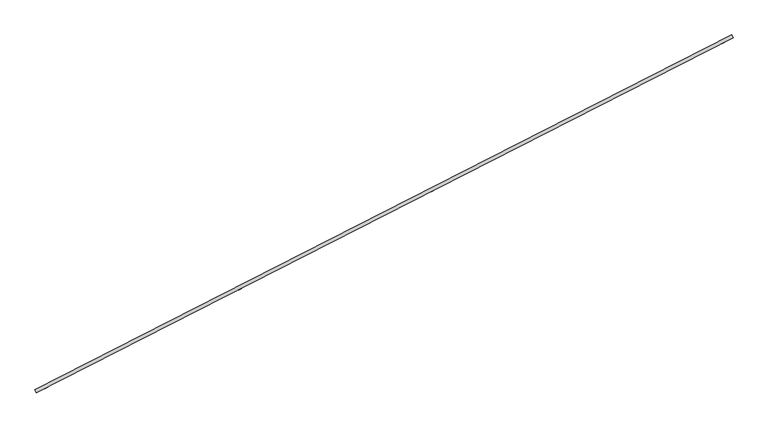
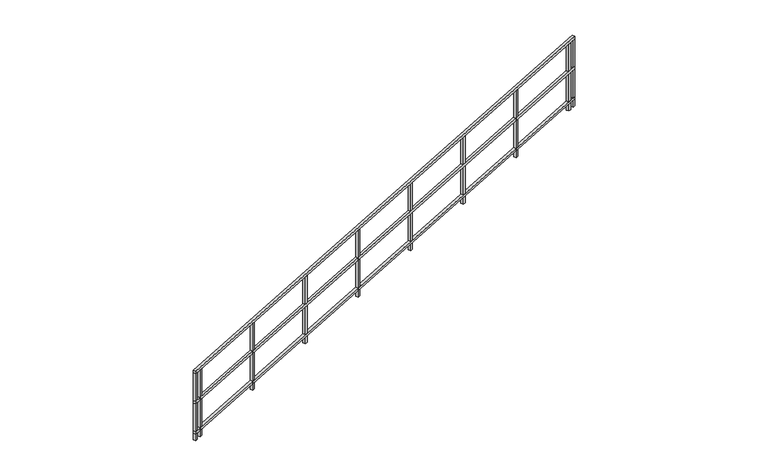
"""IFC4 building model written with IfcOpenShell, lengths in millimetres: railing geometry."""

from ifc_helpers import new_model, si_unit, frame, origin, place, context, project, spatial, polyline, outline, extrude, source, transform, mapped, element, save


def railing_8f82b1fa(model_context):
    return source(origin(), model_context, "Body", "SweptSolid", [
        extrude(outline(polyline([(54203.6748483, 45637.5924682), (54220.9718863, 45603.6451197), (46399.2676625, 41618.2877592), (46381.9706245, 41652.2351078), (54203.6748483, 45637.5924682)])), frame((0.0, 0.0, 266339.5064882), z_axis=(0.0, 0.0, 1.0), x_axis=(1.0, 0.0, 0.0)), (0.0, 0.0, 1.0), 38.1),
        extrude(outline(polyline([(54203.6748483, 45637.5924682), (54220.9718863, 45603.6451197), (46399.2676625, 41618.2877592), (46381.9706245, 41652.2351078), (54203.6748483, 45637.5924682)])), frame((0.0, 0.0, 265875.9564882), z_axis=(0.0, 0.0, 1.0), x_axis=(1.0, 0.0, 0.0)), (0.0, 0.0, 1.0), 38.1),
        extrude(outline(polyline([(54203.6748483, 45637.5924682), (54220.9718863, 45603.6451197), (46399.2676625, 41618.2877592), (46381.9706245, 41652.2351078), (54203.6748483, 45637.5924682)])), frame((0.0, 0.0, 265412.4064882), z_axis=(0.0, 0.0, 1.0), x_axis=(1.0, 0.0, 0.0)), (0.0, 0.0, 1.0), 38.1),
        extrude(outline(polyline([(46524.9904087, 41682.346698), (46491.0430601, 41665.0496599), (46473.7460221, 41698.9970085), (46507.6933706, 41716.2940465), (46524.9904087, 41682.346698)])), frame((0.0, 0.0, 265310.8064882), z_axis=(0.0, 0.0, 1.0), x_axis=(1.0, 0.0, 0.0)), (0.0, 0.0, 1.0), 1028.7),
        extrude(outline(polyline([(47611.305563, 42235.8519153), (47577.3582144, 42218.5548772), (47560.0611764, 42252.5022258), (47594.0085249, 42269.7992638), (47611.305563, 42235.8519153)])), frame((0.0, 0.0, 265310.8064882), z_axis=(0.0, 0.0, 1.0), x_axis=(1.0, 0.0, 0.0)), (0.0, 0.0, 1.0), 1028.7),
        extrude(outline(polyline([(48697.6207173, 42789.3571325), (48663.6733687, 42772.0600945), (48646.3763307, 42806.0074431), (48680.3236792, 42823.3044811), (48697.6207173, 42789.3571325)])), frame((0.0, 0.0, 265310.8064882), z_axis=(0.0, 0.0, 1.0), x_axis=(1.0, 0.0, 0.0)), (0.0, 0.0, 1.0), 1028.7),
        extrude(outline(polyline([(49783.9358716, 43342.8623498), (49749.988523, 43325.5653118), (49732.6914849, 43359.5126604), (49766.6388335, 43376.8096984), (49783.9358716, 43342.8623498)])), frame((0.0, 0.0, 265310.8064882), z_axis=(0.0, 0.0, 1.0), x_axis=(1.0, 0.0, 0.0)), (0.0, 0.0, 1.0), 1028.7),
        extrude(outline(polyline([(50870.2510258, 43896.3675671), (50836.3036773, 43879.0705291), (50819.0066392, 43913.0178776), (50852.9539878, 43930.3149157), (50870.2510258, 43896.3675671)])), frame((0.0, 0.0, 265310.8064882), z_axis=(0.0, 0.0, 1.0), x_axis=(1.0, 0.0, 0.0)), (0.0, 0.0, 1.0), 1028.7),
        extrude(outline(polyline([(51956.5661801, 44449.8727844), (51922.6188316, 44432.5757463), (51905.3217935, 44466.5230949), (51939.2691421, 44483.820133), (51956.5661801, 44449.8727844)])), frame((0.0, 0.0, 265310.8064882), z_axis=(0.0, 0.0, 1.0), x_axis=(1.0, 0.0, 0.0)), (0.0, 0.0, 1.0), 1028.7),
        extrude(outline(polyline([(53042.8813344, 45003.3780017), (53008.9339859, 44986.0809636), (52991.6369478, 45020.0283122), (53025.5842964, 45037.3253502), (53042.8813344, 45003.3780017)])), frame((0.0, 0.0, 265310.8064882), z_axis=(0.0, 0.0, 1.0), x_axis=(1.0, 0.0, 0.0)), (0.0, 0.0, 1.0), 1028.7),
        extrude(outline(polyline([(54129.1964887, 45556.883219), (54095.2491401, 45539.5861809), (54077.9521021, 45573.5335295), (54111.8994507, 45590.8305675), (54129.1964887, 45556.883219)])), frame((0.0, 0.0, 265310.8064882), z_axis=(0.0, 0.0, 1.0), x_axis=(1.0, 0.0, 0.0)), (0.0, 0.0, 1.0), 1028.7),
        extrude(outline(polyline([(46433.2150111, 41635.5847973), (46399.2676625, 41618.2877592), (46381.9706245, 41652.2351078), (46415.9179731, 41669.5321458), (46433.2150111, 41635.5847973)])), frame((0.0, 0.0, 265310.8064882), z_axis=(0.0, 0.0, 1.0), x_axis=(1.0, 0.0, 0.0)), (0.0, 0.0, 1.0), 1028.7),
        extrude(outline(polyline([(54220.9718863, 45603.6451197), (54187.0245377, 45586.3480816), (54169.7274997, 45620.2954302), (54203.6748483, 45637.5924682), (54220.9718863, 45603.6451197)])), frame((0.0, 0.0, 265310.8064882), z_axis=(0.0, 0.0, 1.0), x_axis=(1.0, 0.0, 0.0)), (0.0, 0.0, 1.0), 1028.7),
    ])


if __name__ == "__main__":
    model = new_model("IFC4")
    model_context = context("Model", 3, world=origin())
    ifc_project = project(units=[si_unit("LENGTHUNIT", "METRE", prefix="MILLI")], contexts=[model_context])
    site = spatial("IfcSite", under=ifc_project)
    building = spatial("IfcBuilding", under=site)
    placement = place(None, origin())
    railing_shape = railing_8f82b1fa(model_context)
    element("IfcRailing", 1, at=placement, inside=building, context=model_context, shape_type="MappedRepresentation", body=[
        mapped(railing_shape, transform((0.0, 0.0, 0.0), x_axis=(1.0, 0.0, 0.0), y_axis=(0.0, 1.0, 0.0), z_axis=(0.0, 0.0, 1.0))),
    ])
    save(model, "model.ifc")

# Revit data of these elements
# Element 1 (IfcRailing)
#   Materials on its faces: "Laypere Stair - Powder Coated Steel - Color as Specified"
# Materials
#   "Laypere Stair - Powder Coated Steel - Color as Specified": class "Miscellaneous", colour RGB 178 35 35, transparency 0, Keynote = "05 52 00", Model = "Powder Coated Steel - Color as Specified", Manufacturer = "LAPEYRE STAIR, INC.", Description = "Powder Coated Steel - Color as Specified", Cost = 0
